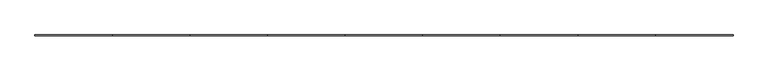
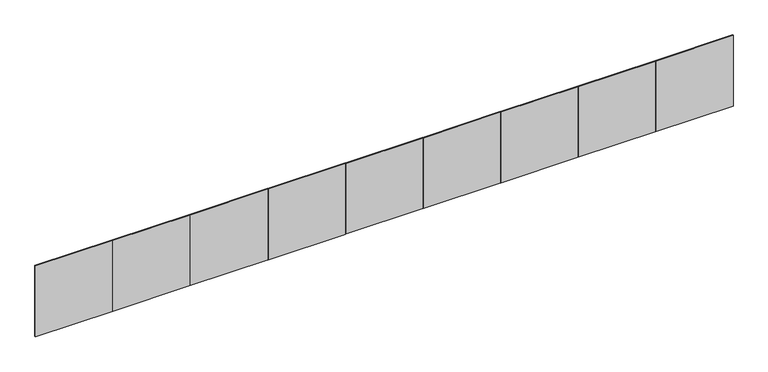
"""IFC4 building model written with IfcOpenShell, lengths in millimetres: railing geometry, ML_Painéis : ML_Painéis."""

from ifc_helpers import new_model, si_unit, frame, origin, place, context, project, spatial, polyline, outline, extrude, source, transform, mapped, element, save


def railing_be0b07b7(model_context):
    return source(origin(), model_context, "Body", "SweptSolid", [
        extrude(outline(polyline([(-4674.5702584, 2133.3602771), (-4674.5702584, 2121.3602771), (-5709.5702584, 2121.3602771), (-5709.5702584, 2133.3602771), (-4674.5702584, 2133.3602771)])), frame((0.0, 0.0, 4122.0679199), z_axis=(0.0, 0.0, 1.0), x_axis=(1.0, 0.0, 0.0)), (0.0, 0.0, 1.0), 1000.0),
        extrude(outline(polyline([(-5711.5702584, 2133.3602771), (-5711.5702584, 2121.3602771), (-6746.5702584, 2121.3602771), (-6746.5702584, 2133.3602771), (-5711.5702584, 2133.3602771)])), frame((0.0, 0.0, 4122.0679199), z_axis=(0.0, 0.0, 1.0), x_axis=(1.0, 0.0, 0.0)), (0.0, 0.0, 1.0), 1000.0),
        extrude(outline(polyline([(-6748.5702584, 2133.3602771), (-6748.5702584, 2121.3602771), (-7783.5702584, 2121.3602771), (-7783.5702584, 2133.3602771), (-6748.5702584, 2133.3602771)])), frame((0.0, 0.0, 4122.0679199), z_axis=(0.0, 0.0, 1.0), x_axis=(1.0, 0.0, 0.0)), (0.0, 0.0, 1.0), 1000.0),
        extrude(outline(polyline([(-7785.5702584, 2133.3602771), (-7785.5702584, 2121.3602771), (-8820.5702584, 2121.3602771), (-8820.5702584, 2133.3602771), (-7785.5702584, 2133.3602771)])), frame((0.0, 0.0, 4122.0679199), z_axis=(0.0, 0.0, 1.0), x_axis=(1.0, 0.0, 0.0)), (0.0, 0.0, 1.0), 1000.0),
        extrude(outline(polyline([(-8822.5702584, 2133.3602771), (-8822.5702584, 2121.3602771), (-9857.5702584, 2121.3602771), (-9857.5702584, 2133.3602771), (-8822.5702584, 2133.3602771)])), frame((0.0, 0.0, 4122.0679199), z_axis=(0.0, 0.0, 1.0), x_axis=(1.0, 0.0, 0.0)), (0.0, 0.0, 1.0), 1000.0),
        extrude(outline(polyline([(-9859.5702584, 2133.3602771), (-9859.5702584, 2121.3602771), (-10894.5702584, 2121.3602771), (-10894.5702584, 2133.3602771), (-9859.5702584, 2133.3602771)])), frame((0.0, 0.0, 4122.0679199), z_axis=(0.0, 0.0, 1.0), x_axis=(1.0, 0.0, 0.0)), (0.0, 0.0, 1.0), 1000.0),
        extrude(outline(polyline([(-10896.5702584, 2133.3602771), (-10896.5702584, 2121.3602771), (-11931.5702584, 2121.3602771), (-11931.5702584, 2133.3602771), (-10896.5702584, 2133.3602771)])), frame((0.0, 0.0, 4122.0679199), z_axis=(0.0, 0.0, 1.0), x_axis=(1.0, 0.0, 0.0)), (0.0, 0.0, 1.0), 1000.0),
        extrude(outline(polyline([(-11933.5702584, 2133.3602771), (-11933.5702584, 2121.3602771), (-12968.5702584, 2121.3602771), (-12968.5702584, 2133.3602771), (-11933.5702584, 2133.3602771)])), frame((0.0, 0.0, 4122.0679199), z_axis=(0.0, 0.0, 1.0), x_axis=(1.0, 0.0, 0.0)), (0.0, 0.0, 1.0), 1000.0),
        extrude(outline(polyline([(-12970.5702584, 2133.3602771), (-12970.5702584, 2121.3602771), (-14005.5702584, 2121.3602771), (-14005.5702584, 2133.3602771), (-12970.5702584, 2133.3602771)])), frame((0.0, 0.0, 4122.0679199), z_axis=(0.0, 0.0, 1.0), x_axis=(1.0, 0.0, 0.0)), (0.0, 0.0, 1.0), 1000.0),
    ])


if __name__ == "__main__":
    model = new_model("IFC4")
    model_context = context("Model", 3, world=origin())
    ifc_project = project(units=[si_unit("LENGTHUNIT", "METRE", prefix="MILLI")], contexts=[model_context])
    site = spatial("IfcSite", under=ifc_project)
    building = spatial("IfcBuilding", under=site)
    placement = place(None, origin())
    railing_shape = railing_be0b07b7(model_context)
    element("IfcRailing", 1, ObjectType="ML_Painéis : ML_Painéis", at=placement, inside=building, context=model_context, shape_type="MappedRepresentation", body=[
        mapped(railing_shape, transform((0.0, 0.0, 0.0), x_axis=(1.0, 0.0, 0.0), y_axis=(0.0, 1.0, 0.0), z_axis=(0.0, 0.0, 1.0))),
    ])
    save(model, "model.ifc")

# Revit data of these elements
# Type "ML_Painéis : ML_Painéis"
#   ME_Área [instance default] = 9.315 m²
#   ME_Espessura [instance default] = 0.012 m
#   ME_Dist Painéis [instance default] = 0.002 m
#   ME_Compr Painéis [instance default] = 1.035 m
#   ME_Compr [instance default] = 9.335 m
#   ME_Altura [instance default] = 1.00 m
#   ME_Quant Painéis [instance default] = 9
#   ME_Painel Único [instance default] = no
#   ME_Paineis Vários [instance default] = yes
#   ME_Material Tipo Vidro [instance default] = .VIDRO GENÉRICO
# Element 1 (IfcRailing, "ML_Painéis : ML_Painéis")
#   Materials on its faces: ".VIDRO GENÉRICO"
# Materials
#   ".VIDRO GENÉRICO": class ".CC_VIDRO", colour RGB 0 128 192, transparency 0.9, Description = "Vidro comum", Cost = 0
